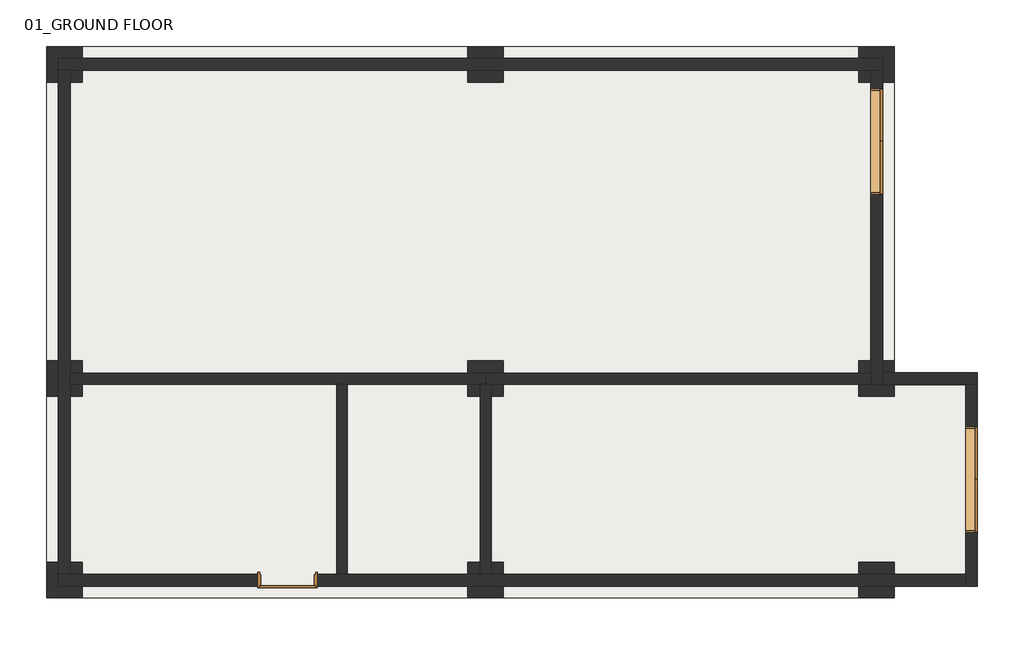
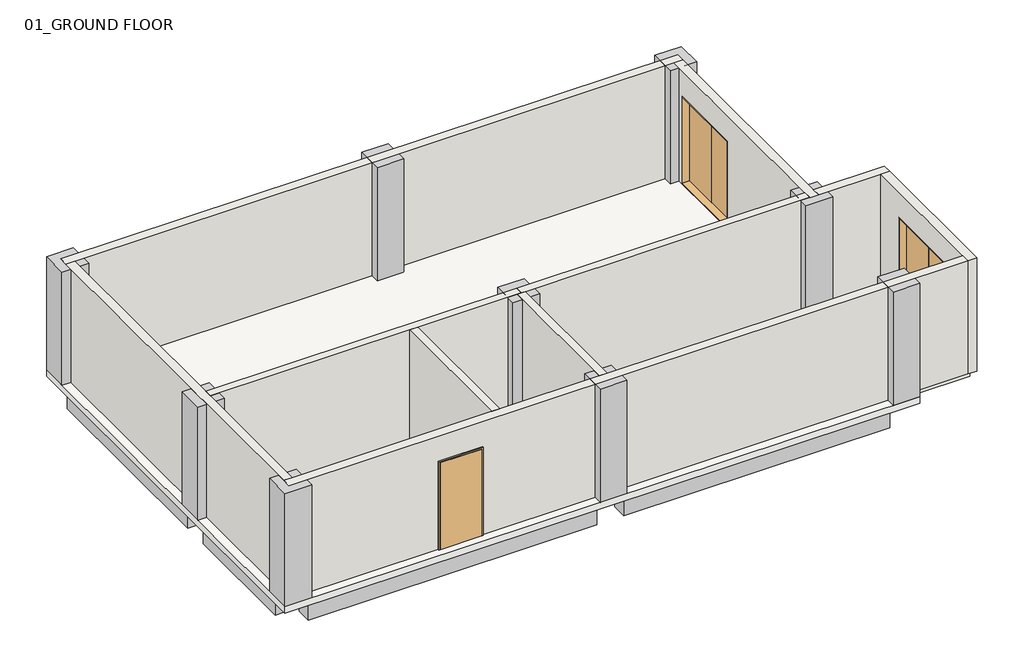
# One storey: 10 walls, 9 columns, 8 beams, 3 doors, 1 slab.
"""IFC4 building model written with IfcOpenShell, lengths in millimetres."""

import ifcopenshell
import ifcopenshell.guid

model = None  # the IFC model being written
_history = None  # IfcOwnerHistory: only IFC2X3 demands one
_inside = {}  # id of a spatial element -> (the spatial element, [elements in it])
_under = {}  # id of a project, library or spatial element -> (it, [spatial elements below it])
_declared = {}  # id of a project -> (the project, [libraries it declares])
_typed = {}  # id of a type object -> (the type object, [elements of that type])
_made_of = {}  # id of a material, layer set ... -> (it, [elements and type objects made of it])


def new_model(schema):
    """Start an empty IFC model of exactly this schema.

    Asked for "IFC4X3", IfcOpenShell would pick the latest addendum, in which some entities
    have other attributes; the version numbers below select the first issue.
    IFC2X3 requires an IfcOwnerHistory on every rooted entity: one is made here for all.
    """
    global model, _history
    if schema == "IFC4X3":
        model = ifcopenshell.file(schema_version=(4, 3, 0, 0))
    else:
        model = ifcopenshell.file(schema=schema)
    _inside.clear()
    _under.clear()
    _declared.clear()
    _typed.clear()
    _made_of.clear()
    _history = None
    if model.schema == "IFC2X3":
        org = make("IfcOrganization", Name="unknown")
        user = make(
            "IfcPersonAndOrganization",
            ThePerson=make("IfcPerson", FamilyName="unknown"),
            TheOrganization=org,
        )
        app = make(
            "IfcApplication",
            ApplicationDeveloper=org,
            Version="unknown",
            ApplicationFullName="unknown",
            ApplicationIdentifier="unknown",
        )
        _history = make(
            "IfcOwnerHistory",
            OwningUser=user,
            OwningApplication=app,
            ChangeAction="ADDED",
            CreationDate=0,
        )
    return model


def make(cls, **values):
    """One entity of the class cls with the attributes given. An attribute that is None is left unset."""
    return model.create_entity(
        cls, **{name: value for name, value in values.items() if value is not None}
    )


def rooted(cls, **values):
    """An entity with a GlobalId (a new one), such as an element, a storey or a relation."""
    return make(cls, GlobalId=ifcopenshell.guid.new(), OwnerHistory=_history, **values)


def si_unit(unit_type, name, prefix=None):
    """IfcSIUnit, for example si_unit("LENGTHUNIT", "METRE", prefix="MILLI")."""
    return make("IfcSIUnit", UnitType=unit_type, Prefix=prefix, Name=name)


def assignment(units):
    """IfcUnitAssignment: the units of a project."""
    return None if units is None else make("IfcUnitAssignment", Units=units)


def point(xyz):
    """IfcCartesianPoint."""
    return None if xyz is None else make("IfcCartesianPoint", Coordinates=xyz)


def direction(xyz):
    """IfcDirection."""
    return None if xyz is None else make("IfcDirection", DirectionRatios=xyz)


def frame(location, z_axis=None, x_axis=None):
    """IfcAxis2Placement3D, a coordinate frame: its origin and axes. An axis left out is left unset."""
    return make(
        "IfcAxis2Placement3D",
        Location=point(location),
        Axis=direction(z_axis),
        RefDirection=direction(x_axis),
    )


def origin():
    """The frame at (0, 0, 0) with its axes left unset."""
    return frame((0.0, 0.0, 0.0))


def origin_with_axes():
    """The frame at (0, 0, 0) with the z axis (0, 0, 1) and the x axis (1, 0, 0) written out."""
    return frame((0.0, 0.0, 0.0), z_axis=(0.0, 0.0, 1.0), x_axis=(1.0, 0.0, 0.0))


def place(relative_to, where):
    """IfcLocalPlacement: puts the frame where relative to a parent placement (None: the world)."""
    return make(
        "IfcLocalPlacement", PlacementRelTo=relative_to, RelativePlacement=where
    )


def context(
    kind, dimensions, precision=None, world=None, true_north=None, identifier=None
):
    """IfcGeometricRepresentationContext, for example the 3D "Model" context."""
    return make(
        "IfcGeometricRepresentationContext",
        ContextIdentifier=identifier,
        ContextType=kind,
        CoordinateSpaceDimension=dimensions,
        Precision=precision,
        WorldCoordinateSystem=world,
        TrueNorth=true_north,
    )


def project(units=None, contexts=None):
    """IfcProject with its units and contexts."""
    return rooted(
        "IfcProject",
        Name="project",
        RepresentationContexts=contexts,
        UnitsInContext=assignment(units),
    )


def spatial(cls, under=None, at=None, **own):
    """A site, building, storey or space (cls), placed at a placement, below another one or the project."""
    s = rooted(cls, ObjectPlacement=at, **own)
    if under is not None:
        _under.setdefault(under.id(), (under, []))[1].append(s)
    return s


def polyline(points):
    """IfcPolyline through the points."""
    return make("IfcPolyline", Points=[point(p) for p in points])


def outline(outer, holes=None, kind="AREA"):
    """IfcArbitraryClosedProfileDef: a profile drawn as a closed curve; with holes, ...WithVoids."""
    if holes is None:
        return make("IfcArbitraryClosedProfileDef", ProfileType=kind, OuterCurve=outer)
    return make(
        "IfcArbitraryProfileDefWithVoids",
        ProfileType=kind,
        OuterCurve=outer,
        InnerCurves=holes,
    )


def extrude(swept, where, along, depth):
    """IfcExtrudedAreaSolid: the profile swept, set in the frame where, extruded along a direction by depth."""
    return make(
        "IfcExtrudedAreaSolid",
        SweptArea=swept,
        Position=where,
        ExtrudedDirection=direction(along),
        Depth=depth,
    )


def faces_of(points, faces, orient=None, outer=None):
    """IfcFace entities. A face is a list of loops; a loop is a list of indices into points, from 0.

    orient and outer hold one flag for each loop. By default every Orientation is true, the
    first loop of a face is its IfcFaceOuterBound and the others are IfcFaceBound.
    """
    made = []
    for i, loops in enumerate(faces):
        bounds = []
        for j, loop in enumerate(loops):
            is_outer = j == 0 if outer is None else outer[i][j]
            bounds.append(
                make(
                    "IfcFaceOuterBound" if is_outer else "IfcFaceBound",
                    Bound=make("IfcPolyLoop", Polygon=[points[k] for k in loop]),
                    Orientation=True if orient is None else orient[i][j],
                )
            )
        made.append(make("IfcFace", Bounds=bounds))
    return made


def faceted_brep(points, faces, orient=None, outer=None, voids=None):
    """IfcFacetedBrep: a solid bounded by flat faces; with voids (closed shells), ...WithVoids."""
    shared = [point(p) for p in points]
    hull = make("IfcClosedShell", CfsFaces=faces_of(shared, faces, orient, outer))
    if voids is None:
        return make("IfcFacetedBrep", Outer=hull)
    return make(
        "IfcFacetedBrepWithVoids",
        Outer=hull,
        Voids=[
            make(cls, CfsFaces=faces_of(shared, fs, o, b)) for cls, fs, o, b in voids
        ],
    )


def shape(context_of_items, identifier, shape_type, items):
    """IfcShapeRepresentation: the items that make up one representation, for example the "Body"."""
    return make(
        "IfcShapeRepresentation",
        ContextOfItems=context_of_items,
        RepresentationIdentifier=identifier,
        RepresentationType=shape_type,
        Items=items,
    )


def source(mapping_origin, context_of_items, identifier, shape_type, items):
    """IfcRepresentationMap: a shape defined once, which mapped items show again and again."""
    return make(
        "IfcRepresentationMap",
        MappingOrigin=mapping_origin,
        MappedRepresentation=shape(context_of_items, identifier, shape_type, items),
    )


def transform(
    local_origin,
    x_axis=None,
    y_axis=None,
    z_axis=None,
    scale=None,
    scale2=None,
    scale3=None,
    uniform=True,
):
    """IfcCartesianTransformationOperator3D, or its non-uniform kind. x_axis, y_axis, z_axis: its Axis1, 2, 3."""
    if uniform:
        return make(
            "IfcCartesianTransformationOperator3D",
            Axis1=direction(x_axis),
            Axis2=direction(y_axis),
            LocalOrigin=point(local_origin),
            Scale=scale,
            Axis3=direction(z_axis),
        )
    return make(
        "IfcCartesianTransformationOperator3DnonUniform",
        Axis1=direction(x_axis),
        Axis2=direction(y_axis),
        LocalOrigin=point(local_origin),
        Scale=scale,
        Axis3=direction(z_axis),
        Scale2=scale2,
        Scale3=scale3,
    )


def mapped(mapping_source, mapping_target):
    """IfcMappedItem: shows the shape of a source again, moved by a transform."""
    return make(
        "IfcMappedItem", MappingSource=mapping_source, MappingTarget=mapping_target
    )


def made_of(thing, what):
    """Note that an element or type object is made of a material, layer set ...; save() writes the relation."""
    if what is not None:
        _made_of.setdefault(what.id(), (what, []))[1].append(thing)
    return thing


def element(
    cls,
    number,
    at=None,
    inside=None,
    cuts=None,
    type_object=None,
    material=None,
    context=None,
    identifier="Body",
    shape_type=None,
    held_by="IfcProductDefinitionShape",
    body=None,
    shapes=None,
    **own,
):
    """One element of the class cls, such as IfcWall. Its Tag is "e" and its number.

    at: its placement. inside: the storey or other place that contains it. cuts: it is an
    opening in that element (IfcRelVoidsElement). A single representation is given by context,
    identifier, shape_type and body (its items); several are given by shapes. held_by: the class
    of the entity that holds the representations. save() writes the other relations.
    """
    e = rooted(cls, Tag="e%d" % number, ObjectPlacement=at, **own)
    if body is not None:
        shapes = [shape(context, identifier, shape_type, body)]
    if shapes is not None:
        e.Representation = make(held_by, Representations=shapes)
    if inside is not None:
        _inside.setdefault(inside.id(), (inside, []))[1].append(e)
    if cuts is not None:
        rooted(
            "IfcRelVoidsElement", RelatingBuildingElement=cuts, RelatedOpeningElement=e
        )
    if type_object is not None:
        _typed.setdefault(type_object.id(), (type_object, []))[1].append(e)
    return made_of(e, material)


def aggregate(whole, parts):
    """IfcRelAggregates: a whole, such as a stair, and the parts it consists of."""
    return rooted("IfcRelAggregates", RelatingObject=whole, RelatedObjects=parts)


def save(model, path):
    """Write the relations noted so far, then the file.

    IfcRelAggregates (storeys below a building ...), IfcRelContainedInSpatialStructure (elements
    in a storey), IfcRelDefinesByType, IfcRelAssociatesMaterial and IfcRelDeclares: one each for
    every whole, place, type object, material and project.
    """
    for whole, parts in _under.values():
        aggregate(whole, parts)
    for where, things in _inside.values():
        rooted(
            "IfcRelContainedInSpatialStructure",
            RelatedElements=things,
            RelatingStructure=where,
        )
    for kind, things in _typed.values():
        rooted("IfcRelDefinesByType", RelatedObjects=things, RelatingType=kind)
    for what, things in _made_of.values():
        rooted("IfcRelAssociatesMaterial", RelatedObjects=things, RelatingMaterial=what)
    for by, libraries in _declared.values():
        rooted("IfcRelDeclares", RelatingContext=by, RelatedDefinitions=libraries)
    model.write(path)


def double_door_steel_22a565f0(model_context):
    return source(origin(), model_context, "Body", "SolidModel", [
        extrude(outline(polyline([(880.0, 60.0), (0.0, 60.0), (0.0, 100.0), (880.0, 100.0), (880.0, 60.0)])), frame((0.0, 0.0, 20.0), z_axis=(0.0, 0.0, 1.0), x_axis=(1.0, 0.0, 0.0)), (0.0, 0.0, 1.0), 2060.0),
        extrude(outline(polyline([(0.0, 60.0), (-880.0, 60.0), (-880.0, 100.0), (0.0, 100.0), (0.0, 60.0)])), frame((0.0, 0.0, 20.0), z_axis=(0.0, 0.0, 1.0), x_axis=(1.0, 0.0, 0.0)), (0.0, 0.0, 1.0), 2060.0),
        faceted_brep([(900.0, -100.0, 2100.0), (900.0, 100.0, 2100.0), (-900.0, 100.0, 2100.0), (-900.0, -100.0, 2100.0), (865.0, 60.0, 2065.0), (865.0, -100.0, 2065.0), (-865.0, -100.0, 2065.0), (-865.0, 60.0, 2065.0), (880.0, 100.0, 2080.0), (880.0, 60.0, 2080.0), (-880.0, 60.0, 2080.0), (-880.0, 100.0, 2080.0), (-900.0, 100.0, 0.0), (-900.0, -100.0, 0.0), (-865.0, -100.0, 35.0), (-865.0, 60.0, 35.0), (-880.0, 60.0, 20.0), (-880.0, 100.0, 20.0), (900.0, 100.0, 0.0), (880.0, 100.0, 20.0), (900.0, -100.0, 0.0), (865.0, -100.0, 35.0), (865.0, 60.0, 35.0), (880.0, 60.0, 20.0)], [[[0, 1, 2, 3]], [[4, 5, 6, 7]], [[8, 9, 10, 11]], [[3, 2, 12, 13]], [[7, 6, 14, 15]], [[11, 10, 16, 17]], [[18, 12, 2, 1], [8, 11, 17, 19]], [[13, 12, 18, 20]], [[0, 3, 13, 20], [21, 14, 6, 5]], [[15, 14, 21, 22]], [[23, 16, 10, 9], [4, 7, 15, 22]], [[17, 16, 23, 19]], [[20, 18, 1, 0]], [[22, 21, 5, 4]], [[19, 23, 9, 8]]]),
    ])


def single_door_steel_4a6c7de9(model_context):
    return source(origin(), model_context, "Body", "SolidModel", [
        extrude(outline(polyline([(470.0, 130.0), (470.0, 95.0), (-470.0, 95.0), (-470.0, 130.0), (470.0, 130.0)])), origin_with_axes(), (0.0, 0.0, 1.0), 2070.0),
        faceted_brep([(470.0, 130.0, 0.0), (500.0, 130.0, 0.0), (500.0, -130.0, 0.0), (470.0, -130.0, 0.0), (470.0, -95.0, 0.0), (450.0, -95.0, 0.0), (450.0, 95.0, 0.0), (470.0, 95.0, 0.0), (470.0, 130.0, 2070.0), (-470.0, 130.0, 2070.0), (-470.0, 130.0, 0.0), (-500.0, 130.0, 0.0), (-500.0, 130.0, 2100.0), (500.0, 130.0, 2100.0), (500.0, -130.0, 2100.0), (-500.0, -130.0, 2100.0), (-500.0, -130.0, 0.0), (-470.0, -130.0, 0.0), (-470.0, -130.0, 2070.0), (470.0, -130.0, 2070.0), (470.0, -95.0, 2070.0), (-470.0, -95.0, 2070.0), (-470.0, -95.0, 0.0), (-450.0, -95.0, 0.0), (-450.0, -95.0, 2050.0), (450.0, -95.0, 2050.0), (450.0, 95.0, 2050.0), (-450.0, 95.0, 2050.0), (-450.0, 95.0, 0.0), (-470.0, 95.0, 0.0), (-470.0, 95.0, 2070.0), (470.0, 95.0, 2070.0)], [[[0, 1, 2, 3, 4, 5, 6, 7]], [[1, 0, 8, 9, 10, 11, 12, 13]], [[2, 1, 13, 14]], [[3, 2, 14, 15, 16, 17, 18, 19]], [[4, 3, 19, 20]], [[5, 4, 20, 21, 22, 23, 24, 25]], [[6, 5, 25, 26]], [[7, 6, 26, 27, 28, 29, 30, 31]], [[0, 7, 31, 8]], [[9, 30, 29, 10]], [[10, 29, 28, 23, 22, 17, 16, 11]], [[15, 12, 11, 16]], [[21, 18, 17, 22]], [[27, 24, 23, 28]], [[14, 13, 12, 15]], [[20, 19, 18, 21]], [[26, 25, 24, 27]], [[8, 31, 30, 9]]]),
    ])


model = new_model("IFC4")

# Units and contexts
model_context = context("Model", 3, world=origin())
ifc_project = project(units=[si_unit("LENGTHUNIT", "METRE", prefix="MILLI")], contexts=[model_context])

# Site, building, storey
site = spatial("IfcSite", under=ifc_project)
building = spatial("IfcBuilding", under=site)
storey = spatial("IfcBuildingStorey", under=building, Name="01_GROUND FLOOR", Elevation=599.9618634)

# Beams
placement = place(None, origin())
element("IfcBeam", 1, ObjectType="RC Beam_Rectangular : H_SB_AR_S16_TG_B400xH600", at=placement, inside=storey, context=model_context, shape_type="SweptSolid", body=[
    extrude(outline(polyline([(13875.0, 1499.5208589), (13525.0, 1499.5208589), (13525.0, 6199.5208589), (13875.0, 6199.5208589), (13875.0, 1499.5208589)])), frame((0.0, 0.0, -0.0381366), z_axis=(0.0, 0.0, 1.0), x_axis=(1.0, 0.0, 0.0)), (0.0, 0.0, 1.0), 450.0),
])
element("IfcBeam", 2, ObjectType="RC Beam_Rectangular : H_SB_AR_S16_TG_B400xH600", at=placement, inside=storey, context=model_context, shape_type="SweptSolid", body=[
    extrude(outline(polyline([(13525.0, 899.5208589), (13875.0, 899.5208589), (13875.0, -1900.4791411), (13525.0, -1900.4791411), (13525.0, 899.5208589)])), frame((0.0, 0.0, -0.0381366), z_axis=(0.0, 0.0, 1.0), x_axis=(1.0, 0.0, 0.0)), (0.0, 0.0, 1.0), 450.0),
])
element("IfcBeam", 3, ObjectType="RC Beam_Rectangular : H_SB_AR_S16_TG_B400xH600", at=placement, inside=storey, context=model_context, shape_type="SweptSolid", body=[
    extrude(outline(polyline([(175.0, 1499.5208589), (-175.0, 1499.5208589), (-175.0, 6199.5208589), (175.0, 6199.5208589), (175.0, 1499.5208589)])), frame((0.0, 0.0, -0.0381366), z_axis=(0.0, 0.0, 1.0), x_axis=(1.0, 0.0, 0.0)), (0.0, 0.0, 1.0), 450.0),
])
element("IfcBeam", 4, ObjectType="RC Beam_Rectangular : H_SB_AR_S16_TG_B400xH600", at=placement, inside=storey, context=model_context, shape_type="SweptSolid", body=[
    extrude(outline(polyline([(-175.0, 899.5208589), (175.0, 899.5208589), (175.0, -1900.4791411), (-175.0, -1900.4791411), (-175.0, 899.5208589)])), frame((0.0, 0.0, -0.0381366), z_axis=(0.0, 0.0, 1.0), x_axis=(1.0, 0.0, 0.0)), (0.0, 0.0, 1.0), 450.0),
])
element("IfcBeam", 5, ObjectType="RC Beam_Rectangular : H_SB_AR_S16_TG_B400xH600", at=placement, inside=storey, context=model_context, shape_type="SweptSolid", body=[
    extrude(outline(polyline([(300.0, 6324.5208589), (300.0, 6674.5208589), (6800.0, 6674.5208589), (6800.0, 6324.5208589), (300.0, 6324.5208589)])), frame((0.0, 0.0, -0.0381366), z_axis=(0.0, 0.0, 1.0), x_axis=(1.0, 0.0, 0.0)), (0.0, 0.0, 1.0), 450.0),
])
element("IfcBeam", 6, ObjectType="RC Beam_Rectangular : H_SB_AR_S16_TG_B400xH600", at=placement, inside=storey, context=model_context, shape_type="SweptSolid", body=[
    extrude(outline(polyline([(13400.0, 6674.5208589), (13400.0, 6324.5208589), (7400.0, 6324.5208589), (7400.0, 6674.5208589), (13400.0, 6674.5208589)])), frame((0.0, 0.0, -0.0381366), z_axis=(0.0, 0.0, 1.0), x_axis=(1.0, 0.0, 0.0)), (0.0, 0.0, 1.0), 450.0),
])
element("IfcBeam", 7, ObjectType="RC Beam_Rectangular : H_SB_AR_S16_TG_B400xH600", at=placement, inside=storey, context=model_context, shape_type="SweptSolid", body=[
    extrude(outline(polyline([(300.0, -2375.4791411), (300.0, -2025.4791411), (6800.0, -2025.4791411), (6800.0, -2375.4791411), (300.0, -2375.4791411)])), frame((0.0, 0.0, -0.0381366), z_axis=(0.0, 0.0, 1.0), x_axis=(1.0, 0.0, 0.0)), (0.0, 0.0, 1.0), 450.0),
])
element("IfcBeam", 8, ObjectType="RC Beam_Rectangular : H_SB_AR_S16_TG_B400xH600", at=placement, inside=storey, context=model_context, shape_type="SweptSolid", body=[
    extrude(outline(polyline([(7400.0, -2375.4791411), (7400.0, -2025.4791411), (13400.0, -2025.4791411), (13400.0, -2375.4791411), (7400.0, -2375.4791411)])), frame((0.0, 0.0, -0.0381366), z_axis=(0.0, 0.0, 1.0), x_axis=(1.0, 0.0, 0.0)), (0.0, 0.0, 1.0), 450.0),
])

# Columns
element("IfcColumn", 9, ObjectType="RC_Column_Rectangular : H_SC_AR_S15_W600xL600", at=placement, inside=storey, context=model_context, shape_type="SweptSolid", body=[
    extrude(outline(polyline([(300.0, 1499.5208589), (300.0, 899.5208589), (-300.0, 899.5208589), (-300.0, 1499.5208589), (300.0, 1499.5208589)])), frame((0.0, 0.0, 599.9618634), z_axis=(0.0, 0.0, 1.0), x_axis=(1.0, 0.0, 0.0)), (0.0, 0.0, 1.0), 2700.0),
])
element("IfcColumn", 10, ObjectType="RC_Column_Rectangular : H_SC_AR_S15_W600xL600", at=placement, inside=storey, context=model_context, shape_type="SweptSolid", body=[
    extrude(outline(polyline([(7400.0, 1499.5208589), (7400.0, 899.5208589), (6800.0, 899.5208589), (6800.0, 1499.5208589), (7400.0, 1499.5208589)])), frame((0.0, 0.0, 599.9618634), z_axis=(0.0, 0.0, 1.0), x_axis=(1.0, 0.0, 0.0)), (0.0, 0.0, 1.0), 2700.0),
])
element("IfcColumn", 11, ObjectType="RC_Column_Rectangular : H_SC_AR_S15_W600xL600", at=placement, inside=storey, context=model_context, shape_type="SweptSolid", body=[
    extrude(outline(polyline([(14000.0, 1499.5208589), (14000.0, 899.5208589), (13400.0, 899.5208589), (13400.0, 1499.5208589), (14000.0, 1499.5208589)])), frame((0.0, 0.0, 599.9618634), z_axis=(0.0, 0.0, 1.0), x_axis=(1.0, 0.0, 0.0)), (0.0, 0.0, 1.0), 2700.0),
])
element("IfcColumn", 12, ObjectType="RC_Column_Rectangular : H_SC_AR_S15_W600xL600", at=placement, inside=storey, context=model_context, shape_type="SweptSolid", body=[
    extrude(outline(polyline([(300.0, 6799.5208589), (300.0, 6199.5208589), (-300.0, 6199.5208589), (-300.0, 6799.5208589), (300.0, 6799.5208589)])), frame((0.0, 0.0, 599.9618634), z_axis=(0.0, 0.0, 1.0), x_axis=(1.0, 0.0, 0.0)), (0.0, 0.0, 1.0), 2700.0),
])
element("IfcColumn", 13, ObjectType="RC_Column_Rectangular : H_SC_AR_S15_W600xL600", at=placement, inside=storey, context=model_context, shape_type="SweptSolid", body=[
    extrude(outline(polyline([(7400.0, 6799.5208589), (7400.0, 6199.5208589), (6800.0, 6199.5208589), (6800.0, 6799.5208589), (7400.0, 6799.5208589)])), frame((0.0, 0.0, 599.9618634), z_axis=(0.0, 0.0, 1.0), x_axis=(1.0, 0.0, 0.0)), (0.0, 0.0, 1.0), 2700.0),
])
element("IfcColumn", 14, ObjectType="RC_Column_Rectangular : H_SC_AR_S15_W600xL600", at=placement, inside=storey, context=model_context, shape_type="SweptSolid", body=[
    extrude(outline(polyline([(14000.0, 6799.5208589), (14000.0, 6199.5208589), (13400.0, 6199.5208589), (13400.0, 6799.5208589), (14000.0, 6799.5208589)])), frame((0.0, 0.0, 599.9618634), z_axis=(0.0, 0.0, 1.0), x_axis=(1.0, 0.0, 0.0)), (0.0, 0.0, 1.0), 2700.0),
])
element("IfcColumn", 15, ObjectType="RC_Column_Rectangular : H_SC_AR_S15_W600xL600", at=placement, inside=storey, context=model_context, shape_type="SweptSolid", body=[
    extrude(outline(polyline([(300.0, -1900.4791411), (300.0, -2500.4791411), (-300.0, -2500.4791411), (-300.0, -1900.4791411), (300.0, -1900.4791411)])), frame((0.0, 0.0, 599.9618634), z_axis=(0.0, 0.0, 1.0), x_axis=(1.0, 0.0, 0.0)), (0.0, 0.0, 1.0), 2700.0),
])
element("IfcColumn", 16, ObjectType="RC_Column_Rectangular : H_SC_AR_S15_W600xL600", at=placement, inside=storey, context=model_context, shape_type="SweptSolid", body=[
    extrude(outline(polyline([(7400.0, -1900.4791411), (7400.0, -2500.4791411), (6800.0, -2500.4791411), (6800.0, -1900.4791411), (7400.0, -1900.4791411)])), frame((0.0, 0.0, 599.9618634), z_axis=(0.0, 0.0, 1.0), x_axis=(1.0, 0.0, 0.0)), (0.0, 0.0, 1.0), 2700.0),
])
element("IfcColumn", 17, ObjectType="RC_Column_Rectangular : H_SC_AR_S15_W600xL600", at=placement, inside=storey, context=model_context, shape_type="SweptSolid", body=[
    extrude(outline(polyline([(14000.0, -1900.4791411), (14000.0, -2500.4791411), (13400.0, -2500.4791411), (13400.0, -1900.4791411), (14000.0, -1900.4791411)])), frame((0.0, 0.0, 599.9618634), z_axis=(0.0, 0.0, 1.0), x_axis=(1.0, 0.0, 0.0)), (0.0, 0.0, 1.0), 2700.0),
])

# Doors
double_door_steel_shape = double_door_steel_22a565f0(model_context)
element("IfcDoor", 18, ObjectType="Double Door_Steel : H_DR_AR_B12_Double Door_Steel_W2000xH2100", at=placement, inside=storey, context=model_context, shape_type="MappedRepresentation", body=[
    mapped(double_door_steel_shape, transform((15300.0, -500.4791411, 599.9618634), x_axis=(0.0, -1.0, 0.0), y_axis=(1.0, 0.0, 0.0), z_axis=(0.0, 0.0, 1.0))),
])
element("IfcDoor", 19, ObjectType="Double Door_Steel : H_DR_AR_B12_Double Door_Steel_W2000xH2100", at=placement, inside=storey, context=model_context, shape_type="MappedRepresentation", body=[
    mapped(double_door_steel_shape, transform((13700.0, 5199.5208589, 599.9618634), x_axis=(0.0, -1.0, 0.0), y_axis=(1.0, 0.0, 0.0), z_axis=(0.0, 0.0, 1.0))),
])
single_door_steel_shape = single_door_steel_4a6c7de9(model_context)
element("IfcDoor", 20, ObjectType="Single Door_Steel : H_DR_AR_B12_Single Door_Steel_W1000xH2100", at=placement, inside=storey, context=model_context, shape_type="MappedRepresentation", body=[
    mapped(single_door_steel_shape, transform((3766.0, -2200.4791411, 599.9618634), x_axis=(-1.0, 0.0, 0.0), y_axis=(0.0, -1.0, 0.0), z_axis=(0.0, 0.0, 1.0))),
])

# Slab
element("IfcSlab", 21, ObjectType="H_FL_AR_S17_RC Slab T150", at=placement, inside=storey, context=model_context, shape_type="SweptSolid", body=[
    extrude(outline(polyline([(14000.0, 1199.5208589), (15300.0, 1199.5208589), (15300.0, -2200.4791411), (14000.0, -2200.4791411), (14000.0, -2500.4791411), (-300.0, -2500.4791411), (-300.0, 6799.5208589), (14000.0, 6799.5208589), (14000.0, 1199.5208589)])), frame((0.0, 0.0, 449.9618634), z_axis=(0.0, 0.0, 1.0), x_axis=(1.0, 0.0, 0.0)), (0.0, 0.0, 1.0), 150.0),
])

# Walls
element("IfcWall", 22, ObjectType="H_WA_AR_B02_Ext Wall_RC T200", at=placement, inside=storey, context=model_context, shape_type="Brep", body=[
    faceted_brep([(-100.0, 6399.5208589, 599.9618634), (100.0, 6399.5208589, 599.9618634), (13600.0, 6399.5208589, 599.9618634), (13800.0, 6399.5208589, 599.9618634), (13800.0, 6399.5208589, 3299.9618634), (13600.0, 6399.5208589, 3299.9618634), (100.0, 6399.5208589, 3299.9618634), (-100.0, 6399.5208589, 3299.9618634), (-100.0, 6599.5208589, 599.9618634), (-100.0, 6599.5208589, 3299.9618634), (13800.0, 6599.5208589, 3299.9618634), (13800.0, 6599.5208589, 599.9618634)], [[[0, 1, 2, 3, 4, 5, 6, 7]], [[8, 9, 10, 11]], [[3, 2, 1, 0, 8, 11]], [[7, 6, 5, 4, 10, 9]], [[4, 3, 11, 10]], [[0, 7, 9, 8]]]),
])
element("IfcWall", 23, ObjectType="H_WA_AR_B02_Ext Wall_RC T200", at=placement, inside=storey, context=model_context, shape_type="Brep", body=[
    faceted_brep([(13600.0, 1099.5208589, 3299.9618634), (13600.0, 1102.5208589, 3299.9618634), (13600.0, 1286.5208589, 3299.9618634), (13600.0, 6399.5208589, 3299.9618634), (13600.0, 6399.5208589, 599.9618634), (13600.0, 6099.5208589, 599.9618634), (13600.0, 6099.5208589, 2699.9618634), (13600.0, 4299.5208589, 2699.9618634), (13600.0, 4299.5208589, 599.9618634), (13600.0, 1286.5208589, 599.9618634), (13600.0, 1102.5208589, 599.9618634), (13600.0, 1099.5208589, 599.9618634), (13800.0, 6399.5208589, 3299.9618634), (13800.0, 1299.5208589, 3299.9618634), (13800.0, 1099.5208589, 3299.9618634), (13800.0, 1099.5208589, 599.9618634), (13800.0, 1299.5208589, 599.9618634), (13800.0, 4299.5208589, 599.9618634), (13800.0, 4299.5208589, 2699.9618634), (13800.0, 6099.5208589, 2699.9618634), (13800.0, 6099.5208589, 599.9618634), (13800.0, 6399.5208589, 599.9618634)], [[[0, 1, 2, 3, 4, 5, 6, 7, 8, 9, 10, 11]], [[12, 13, 14, 15, 16, 17, 18, 19, 20, 21]], [[4, 21, 20, 5]], [[15, 11, 10, 9, 8, 17, 16]], [[3, 2, 1, 0, 14, 13, 12]], [[4, 3, 12, 21]], [[0, 11, 15, 14]], [[7, 18, 17, 8]], [[18, 7, 6, 19]], [[19, 6, 5, 20]]]),
])
element("IfcWall", 24, ObjectType="H_WA_AR_B02_Ext Wall_RC T200", at=placement, inside=storey, context=model_context, shape_type="Brep", body=[
    faceted_brep([(13800.0, 1099.5208589, 599.9618634), (15200.0, 1099.5208589, 599.9618634), (15400.0, 1099.5208589, 599.9618634), (15400.0, 1099.5208589, 3299.9618634), (15200.0, 1099.5208589, 3299.9618634), (13800.0, 1099.5208589, 3299.9618634), (13800.0, 1299.5208589, 599.9618634), (13800.0, 1299.5208589, 3299.9618634), (15400.0, 1299.5208589, 3299.9618634), (15400.0, 1299.5208589, 599.9618634)], [[[0, 1, 2, 3, 4, 5]], [[6, 7, 8, 9]], [[2, 1, 0, 6, 9]], [[5, 4, 3, 8, 7]], [[0, 5, 7, 6]], [[3, 2, 9, 8]]]),
])
element("IfcWall", 25, ObjectType="H_WA_AR_B02_Ext Wall_RC T200", at=placement, inside=storey, context=model_context, shape_type="Brep", body=[
    faceted_brep([(15200.0, -2300.4791411, 3299.9618634), (15200.0, -2100.4791411, 3299.9618634), (15200.0, 1099.5208589, 3299.9618634), (15200.0, 1099.5208589, 599.9618634), (15200.0, 399.5208589, 599.9618634), (15200.0, 399.5208589, 2699.9618634), (15200.0, -1400.4791411, 2699.9618634), (15200.0, -1400.4791411, 599.9618634), (15200.0, -2100.4791411, 599.9618634), (15200.0, -2300.4791411, 599.9618634), (15400.0, 1099.5208589, 3299.9618634), (15400.0, -2300.4791411, 3299.9618634), (15400.0, -2300.4791411, 599.9618634), (15400.0, -1400.4791411, 599.9618634), (15400.0, -1400.4791411, 2699.9618634), (15400.0, 399.5208589, 2699.9618634), (15400.0, 399.5208589, 599.9618634), (15400.0, 1099.5208589, 599.9618634)], [[[0, 1, 2, 3, 4, 5, 6, 7, 8, 9]], [[10, 11, 12, 13, 14, 15, 16, 17]], [[3, 17, 16, 4]], [[12, 9, 8, 7, 13]], [[2, 1, 0, 11, 10]], [[3, 2, 10, 17]], [[0, 9, 12, 11]], [[6, 14, 13, 7]], [[14, 6, 5, 15]], [[15, 5, 4, 16]]]),
])
element("IfcWall", 26, ObjectType="H_WA_AR_B02_Ext Wall_RC T200", at=placement, inside=storey, context=model_context, shape_type="Brep", body=[
    faceted_brep([(-100.0, -2100.4791411, 3299.9618634), (100.0, -2100.4791411, 3299.9618634), (4591.0, -2100.4791411, 3299.9618634), (4775.0, -2100.4791411, 3299.9618634), (7013.0, -2100.4791411, 3299.9618634), (7197.0, -2100.4791411, 3299.9618634), (15200.0, -2100.4791411, 3299.9618634), (15200.0, -2100.4791411, 599.9618634), (7197.0, -2100.4791411, 599.9618634), (7013.0, -2100.4791411, 599.9618634), (4775.0, -2100.4791411, 599.9618634), (4591.0, -2100.4791411, 599.9618634), (4266.0, -2100.4791411, 599.9618634), (4266.0, -2100.4791411, 2699.9618634), (3266.0, -2100.4791411, 2699.9618634), (3266.0, -2100.4791411, 599.9618634), (100.0, -2100.4791411, 599.9618634), (-100.0, -2100.4791411, 599.9618634), (15200.0, -2300.4791411, 3299.9618634), (-100.0, -2300.4791411, 3299.9618634), (-100.0, -2300.4791411, 599.9618634), (3266.0, -2300.4791411, 599.9618634), (3266.0, -2300.4791411, 2699.9618634), (4266.0, -2300.4791411, 2699.9618634), (4266.0, -2300.4791411, 599.9618634), (15200.0, -2300.4791411, 599.9618634)], [[[0, 1, 2, 3, 4, 5, 6, 7, 8, 9, 10, 11, 12, 13, 14, 15, 16, 17]], [[18, 19, 20, 21, 22, 23, 24, 25]], [[7, 25, 24, 12, 11, 10, 9, 8]], [[20, 17, 16, 15, 21]], [[6, 5, 4, 3, 2, 1, 0, 19, 18]], [[7, 6, 18, 25]], [[0, 17, 20, 19]], [[14, 22, 21, 15]], [[22, 14, 13, 23]], [[23, 13, 12, 24]]]),
])
element("IfcWall", 27, ObjectType="H_WA_AR_B02_Ext Wall_RC T200", at=placement, inside=storey, context=model_context, shape_type="Brep", body=[
    faceted_brep([(100.0, -2100.4791411, 599.9618634), (100.0, 1102.5208589, 599.9618634), (100.0, 1286.5208589, 599.9618634), (100.0, 6399.5208589, 599.9618634), (100.0, 6399.5208589, 3299.9618634), (100.0, 1286.5208589, 3299.9618634), (100.0, 1102.5208589, 3299.9618634), (100.0, -2100.4791411, 3299.9618634), (-100.0, -2100.4791411, 599.9618634), (-100.0, -2100.4791411, 3299.9618634), (-100.0, 6399.5208589, 3299.9618634), (-100.0, 6399.5208589, 599.9618634)], [[[0, 1, 2, 3, 4, 5, 6, 7]], [[8, 9, 10, 11]], [[3, 2, 1, 0, 8, 11]], [[7, 6, 5, 4, 10, 9]], [[0, 7, 9, 8]], [[4, 3, 11, 10]]]),
])
element("IfcWall", 28, ObjectType="H_WA_AR_B02_Int Wall_Block T150", at=placement, inside=storey, context=model_context, shape_type="Brep", body=[
    faceted_brep([(100.0, 1102.5208589, 599.9618634), (4591.0, 1102.5208589, 599.9618634), (4775.0, 1102.5208589, 599.9618634), (7105.0, 1102.5208589, 599.9618634), (7105.0, 1102.5208589, 3299.9618634), (4775.0, 1102.5208589, 3299.9618634), (4591.0, 1102.5208589, 3299.9618634), (100.0, 1102.5208589, 3299.9618634), (100.0, 1286.5208589, 599.9618634), (100.0, 1286.5208589, 3299.9618634), (7105.0, 1286.5208589, 3299.9618634), (7105.0, 1286.5208589, 599.9618634)], [[[0, 1, 2, 3, 4, 5, 6, 7]], [[8, 9, 10, 11]], [[3, 2, 1, 0, 8, 11]], [[4, 3, 11, 10]], [[7, 6, 5, 4, 10, 9]], [[0, 7, 9, 8]]]),
])
element("IfcWall", 29, ObjectType="H_WA_AR_B02_Int Wall_Block T150", at=placement, inside=storey, context=model_context, shape_type="Brep", body=[
    faceted_brep([(7197.0, -2100.4791411, 599.9618634), (7197.0, 1102.5208589, 599.9618634), (7197.0, 1102.5208589, 3299.9618634), (7197.0, -2100.4791411, 3299.9618634), (7013.0, -2100.4791411, 599.9618634), (7013.0, -2100.4791411, 3299.9618634), (7013.0, 1102.5208589, 3299.9618634), (7013.0, 1102.5208589, 599.9618634), (7105.0, 1102.5208589, 599.9618634), (7105.0, 1102.5208589, 3299.9618634)], [[[0, 1, 2, 3]], [[4, 5, 6, 7]], [[1, 0, 4, 7, 8]], [[3, 2, 9, 6, 5]], [[0, 3, 5, 4]], [[2, 1, 8, 7, 6, 9]]]),
])
element("IfcWall", 30, ObjectType="H_WA_AR_B02_Int Wall_Block T150", at=placement, inside=storey, context=model_context, shape_type="SweptSolid", body=[
    extrude(outline(polyline([(4591.0, -2100.4791411), (4591.0, 1102.5208589), (4775.0, 1102.5208589), (4775.0, -2100.4791411), (4591.0, -2100.4791411)])), frame((0.0, 0.0, 599.9618634), z_axis=(0.0, 0.0, 1.0), x_axis=(1.0, 0.0, 0.0)), (0.0, 0.0, 1.0), 2700.0),
])
element("IfcWall", 31, ObjectType="H_WA_AR_B02_Int Wall_Block T150", at=placement, inside=storey, context=model_context, shape_type="Brep", body=[
    faceted_brep([(7105.0, 1102.5208589, 599.9618634), (7197.0, 1102.5208589, 599.9618634), (13600.0, 1102.5208589, 599.9618634), (13600.0, 1102.5208589, 3299.9618634), (7197.0, 1102.5208589, 3299.9618634), (7105.0, 1102.5208589, 3299.9618634), (7105.0, 1286.5208589, 599.9618634), (7105.0, 1286.5208589, 3299.9618634), (13600.0, 1286.5208589, 3299.9618634), (13600.0, 1286.5208589, 599.9618634)], [[[0, 1, 2, 3, 4, 5]], [[6, 7, 8, 9]], [[2, 1, 0, 6, 9]], [[5, 4, 3, 8, 7]], [[0, 5, 7, 6]], [[3, 2, 9, 8]]]),
])

save(model, "model.ifc")

# Revit data of these elements
# Project information
#   H_Seismic Condition = "A as per ASCE 7-10"
#   H_Soil Condition = "C as per ASCE 7-10"
#   H_Basic Wind Speed = "58.3m/s ASCE7-10"
#   H_DS Project Code = "FAASA2302"
#   H_Project Abbreviation = "SACE2"
#   H_Project Division = "화공"
#   H_Project Finish = "2027-03-05"
#   H_Project Location = "Jafurah, Saudi Arabia"
#   H_Project Start = "2024-01-03"
#   H_Project Type = "EPC"
#   H_Smart Code = "FAASA2302"
#   Project Issue Date = "Issue Date"
#   Project Status = "Project Status"
#   Client Name = "Owner"
#   Project Address = "Enter address here"
#   Project Name = "Project Name"
#   Project Number = "0001"
# Grids (mm)
#   "Y3": line (-3860.098, -2200.479) -> (23085.93, -2200.479)
#   "Y5": line (10022, 8528.879) -> (10022, -4208.346)
#   "Y4": line (3593, 8528.879) -> (3593, -4208.346)
#   "Y6": line (5412.5, 8528.879) -> (5412.5, -4208.346)
#   "Y2": line (-3860.098, 1199.521) -> (23085.93, 1199.521)
#   "X1": line (0, 11877.337) -> (0, -4208.346)
#   "X2": line (7100, 11877.337) -> (7100, -4208.346)
#   "Y1": line (-3860.098, 6499.521) -> (23085.93, 6499.521)
#   "X3": line (13700, 11877.337) -> (13700, -4208.346)
# Type "RC Beam_Rectangular : H_SB_AR_S16_TG_B400xH600"
#   중앙부 하부근 = ""
#   중앙부 상부근 = ""
#   중앙부 보조근 = ""
#   중앙부 늑근 = ""
#   외단부 하부근 = ""
#   외단부 상부근 = ""
#   외단부 보조근 = ""
#   외단부 늑근 = ""
#   부호 = "TG2"
#   내단부 하부근 = ""
#   내단부 상부근 = ""
#   내단부 보조근 = ""
#   내단부 늑근 = ""
#   ALL 하부근 = "3-D20"
#   ALL 상부근 = "4-D20"
#   ALL 보조근 = ""
#   ALL 늑근 = "2-D10 @120"
#   Width = 350 mm
#   Height = 600 mm
#   Length [instance default] = 1524 mm
#   b = 350 mm
#   h = 600 mm
#   hec_material3 [instance default] = none
#   hec_material2 [instance default] = none
#   hec_material1 [instance default] = none
#   Structural Material [instance default] = none
#   Assembly Code = ""
# Type "RC_Column_Rectangular : H_SC_AR_S15_W600xL600"
#   Width = 600 mm
#   Length = 600 mm
#   hec_material3 [instance default] = none
#   hec_material2 [instance default] = none
#   hec_material1 [instance default] = none
#   Structural Material [instance default] = none
#   Description = (empty or 0)
# Type "Double Door_Steel : H_DR_AR_B12_Double Door_Steel_W2000xH2100"
#   Type Mark = ""
#   프레임 = ""
#   철물 = ""
#   유리/마감 = ""
#   위치/개소 = ""
#   부호 = "1/SD"
#   문번호 = ""
#   문기호 = "SD"
#   Analytic Construction = "<None>"
#   Height = 2100 mm
#   Width = 1800 mm
#   Define Thermal Properties by = 1
#   문 틀 = none
#   문 = none
#   Function = (empty or 0)
#   Assembly Code = ""
#   Wall Closure = (empty or 0)
# Type "Single Door_Steel : H_DR_AR_B12_Single Door_Steel_W1000xH2100"
#   Type Mark = "SD"
#   Analytic Construction = "<None>"
#   프레임 투영 외부. = 25 mm
#   프레임 투영 내부. = 25 mm
#   프레임 폭 = 75 mm
#   Height = 2100 mm
#   Width = 1000 mm
#   Define Thermal Properties by = 1
#   문 패널 = none
#   문 프레임 = none
#   Function = (empty or 0)
#   Wall Closure = (empty or 0)
# Type "H_FL_AR_S17_RC Slab T150"
#   Keynote = ""
#   Type Comments = ""
#   Description = ""
#   Function = 1
#   Layers, outside or top first: 150 mm no material (function 1)
# Type "H_WA_AR_B02_Ext Wall_RC T200"
#   Type Comments = ""
#   Layers, outside or top first: 0 mm no material (function 100); 0 mm no material (function 100); 200 mm no material (function 1); 0 mm no material (function 100); 0 mm no material (function 100); 0 mm no material (function 100)
# Type "H_WA_AR_B02_Int Wall_Block T150"
#   Type Comments = ""
#   Layers, outside or top first: 0 mm no material (function 100); 12 mm no material (function 2); 150 mm no material (function 1); 12 mm no material (function 2); 10 mm no material (function 5)
# Elements 1, 2, 3, 4, 5, 6, 7, 8 (IfcBeam, "RC Beam_Rectangular : H_SB_AR_S16_TG_B400xH600")
#   Comments = ""
#   hec_material3 = none
#   hec_material2 = none
#   hec_material1 = none
#   Structural Material = none
#   Phase Created = New Construction
# Elements 9, 10, 11, 12, 13, 14, 15, 16, 17 (IfcColumn, "RC_Column_Rectangular : H_SC_AR_S15_W600xL600")
#   Comments = ""
#   hec_material3 = none
#   hec_material2 = none
#   hec_material1 = none
#   Structural Material = none
#   Phase Created = New Construction
# Elements 18, 19 (IfcDoor, "Double Door_Steel : H_DR_AR_B12_Double Door_Steel_W2000xH2100")
#   Phase Created = New Construction
# Element 20 (IfcDoor, "Single Door_Steel : H_DR_AR_B12_Single Door_Steel_W1000xH2100")
#   Phase Created = New Construction
# Element 21 (IfcSlab, "H_FL_AR_S17_RC Slab T150")
#   Height Offset From Level = 0 mm
#   Phase Created = New Construction
#   Materials on its faces: "Default Floor"
# Elements 22, 23, 24, 25, 26, 27 (IfcWall, "H_WA_AR_B02_Ext Wall_RC T200")
#   Top Offset = 0 mm
#   Base Offset = 0 mm
#   wall height = 2700 mm
#   Phase Created = New Construction
#   Base Constraint = 01_GROUND FLOOR
#   Top Constraint = 02_FIRST FLOOR
#   Materials on its faces: "Default Wall"
# Elements 28, 29, 30, 31 (IfcWall, "H_WA_AR_B02_Int Wall_Block T150")
#   Top Offset = 0 mm
#   Base Offset = 0 mm
#   wall height = 2700 mm
#   Phase Created = New Construction
#   Base Constraint = 01_GROUND FLOOR
#   Top Constraint = 02_FIRST FLOOR
#   Materials on its faces: "Default Wall"
# Materials
#   "Default Floor": class "Miscellaneous", colour RGB 80 80 80, transparency 0
#   "Default Wall": class "Miscellaneous", colour RGB 80 80 80, transparency 0
# Room at (5894, -502.979) mm, phase "New Construction", upper level "02_FIRST FLOOR", upper offset 1000 mm, lower offset -1000 mm
#   Comments = ""
#   Number = "126"
#   Name = "TECHNICAL TOWER"
# Room at (2341.5, -502.979) mm, phase "New Construction", upper level "02_FIRST FLOOR", upper offset 1000 mm, lower offset -1000 mm
#   Comments = ""
#   Number = "127"
#   Name = "CONTROL ROOM"
# Room at (6850, 3847.021) mm, phase "New Construction", upper level "02_FIRST FLOOR", upper offset 1000 mm, lower offset -1000 mm
#   Comments = ""
#   Number = "128"
#   Name = "BREATHING APPARATUS GALLERY"
# Room at (11202.5, -500.479) mm, phase "New Construction", upper level "02_FIRST FLOOR", upper offset 1000 mm, lower offset -1000 mm
#   Comments = ""
#   Number = "129"
#   Name = "STAIRS"
